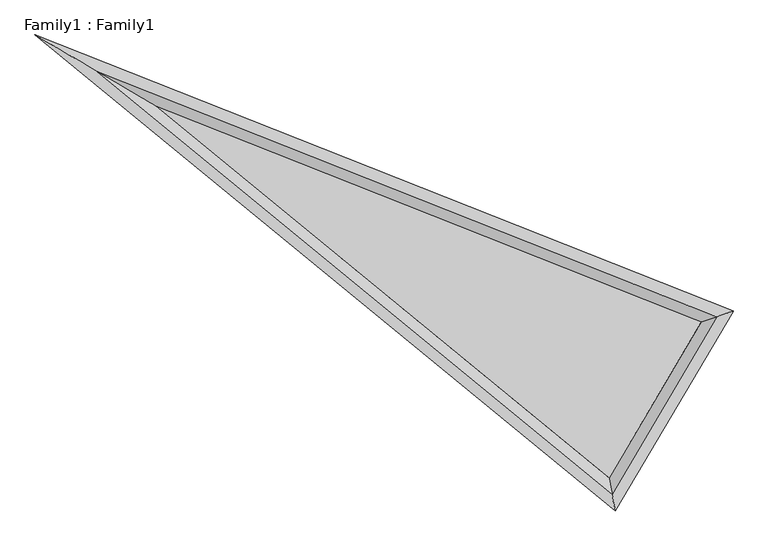
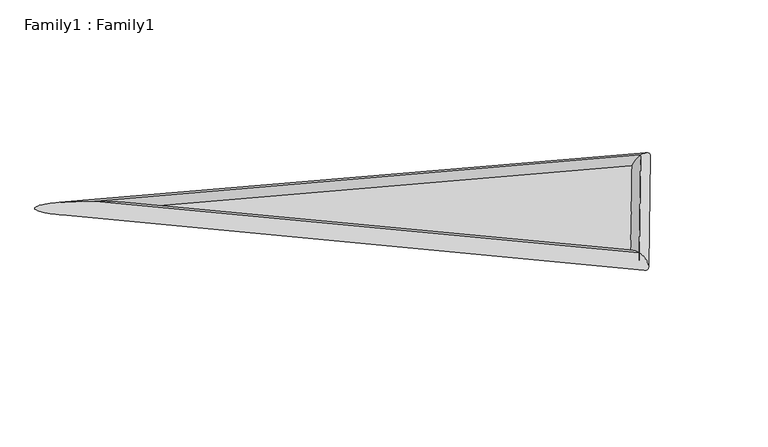
"""IFC4 building model written with IfcOpenShell, lengths in millimetres: proxy geometry, Family1 : Family1."""

from ifc_helpers import new_model, si_unit, frame, origin, origin_with_axes, place, context, project, spatial, polyline, ellipse_curve, outline, extrude, source, transform, mapped, element, save
from ifc_brep_helpers import cylinder_surface, advanced_brep


def family1_family1_00e2fbce(model_context):
    return source(origin(), model_context, "Body", "SolidModel", [
        extrude(outline(polyline([(2142.9027512, -1323.7266856), (-2451.2618622, 2448.6527678), (3075.2815619, 259.0151227), (2142.9027512, -1323.7266856)])), origin_with_axes(), (0.0, 0.0, 1.0), 34.1328789),
        advanced_brep(
        [(2142.9027512, -1323.7266856, 100.0), (2142.9027512, -1323.7266856, -100.0), (-2451.2618622, 2448.6527678, -100.0), (-2451.2618622, 2448.6527678, 100.0), (3075.2815619, 259.0151227, -100.0), (3075.2815619, 259.0151227, 100.0)],
        [
            (0, 1, ellipse_curve(frame((2142.9027512, -1323.7266856, 0.0), z_axis=(-0.9846439546772103, -0.17457457580536712, 0.0), x_axis=(0.17457457580536698, -0.9846439546772103, 0.0)), 153.8014303, 100.0)),
            (1, 2),
            (2, 3, ellipse_curve(frame((-2451.2618622, 2448.6527678, 0.0), z_axis=(-0.5075677185917218, -0.8616118679797734, 0.0), x_axis=(0.8616118679797735, -0.5075677185917219, 0.0)), 647.2135955, 100.0)),
            (3, 0),
            (1, 0, ellipse_curve(frame((2142.9027512, -1323.7266856, 0.0), z_axis=(-0.9846439546772103, -0.17457457580536712, 0.0), x_axis=(0.17457457580536698, -0.9846439546772103, 0.0)), 153.8014303, 100.0)),
            (3, 2, ellipse_curve(frame((-2451.2618622, 2448.6527678, 0.0), z_axis=(-0.5075677185917218, -0.8616118679797734, 0.0), x_axis=(0.8616118679797735, -0.5075677185917219, 0.0)), 647.2135955, 100.0)),
            (2, 4),
            (4, 5, ellipse_curve(frame((3075.2815619, 259.0151227, 0.0), z_axis=(-0.3246140476656981, 0.9458465626400996, 0.0), x_axis=(-0.9458465626400996, -0.32461404766569807, 0.0)), 153.8014303, 100.0)),
            (5, 3),
            (5, 4, ellipse_curve(frame((3075.2815619, 259.0151227, 0.0), z_axis=(-0.3246140476656981, 0.9458465626400996, 0.0), x_axis=(-0.9458465626400996, -0.32461404766569807, 0.0)), 153.8014303, 100.0)),
            (4, 1),
            (0, 5),
        ],
        [
            cylinder_surface(frame((2142.9027512, -1323.7266856, 0.0), z_axis=(0.7728416416572306, -0.6345989260316762, 0.0), x_axis=(-0.6345989260316762, -0.7728416416572306, 0.0)), 100.0),
            cylinder_surface(frame((-2451.2618622, 2448.6527678, 0.0), z_axis=(-0.9296886924981892, 0.36834621627079006, 0.0), x_axis=(0.36834621627079006, 0.9296886924981892, 0.0)), 100.0),
            cylinder_surface(frame((3075.2815619, 259.0151227, 0.0), z_axis=(0.507567718591722, 0.8616118679797734, 0.0), x_axis=(0.8616118679797734, -0.507567718591722, 0.0)), 100.0),
        ],
        [
            (0, [[1, 2, 3, 4]]),
            (0, [[5, -4, 6, -2]]),
            (1, [[-3, 7, 8, 9]]),
            (1, [[-6, -9, 10, -7]]),
            (2, [[-8, 11, -1, 12]]),
            (2, [[-10, -12, -5, -11]]),
        ],
    ),
    ])


if __name__ == "__main__":
    model = new_model("IFC4")
    model_context = context("Model", 3, world=origin())
    ifc_project = project(units=[si_unit("LENGTHUNIT", "METRE", prefix="MILLI")], contexts=[model_context])
    site = spatial("IfcSite", under=ifc_project)
    building = spatial("IfcBuilding", under=site)
    placement = place(None, origin())
    family1_family1_shape = family1_family1_00e2fbce(model_context)
    element("IfcBuildingElementProxy", 1, Name="Family1 : Family1", ObjectType="Family1 : Family1", at=placement, inside=building, context=model_context, shape_type="MappedRepresentation", body=[
        mapped(family1_family1_shape, transform((0.0, 0.0, 0.0), x_axis=(1.0, 0.0, 0.0), y_axis=(0.0, 1.0, 0.0), z_axis=(0.0, 0.0, 1.0))),
    ])
    save(model, "model.ifc")

# Revit data of these elements
# Project information
#   Project Issue Date = "Issue Date"
#   Project Status = "Project Status"
#   Client Name = "Owner"
#   Project Address = "Enter address here"
#   Project Name = "Project Name"
#   Project Number = "0001"
# Type "Family1 : Family1"
#   Default Elevation = 0
# Element 1 (IfcBuildingElementProxy, "Family1 : Family1")
#   Materials on its faces: "Glass"
# Materials
#   "Glass": class "Glass", colour RGB 0 128 192, transparency 0.9, Description = "Soda Lime Glass", Cost = 0
